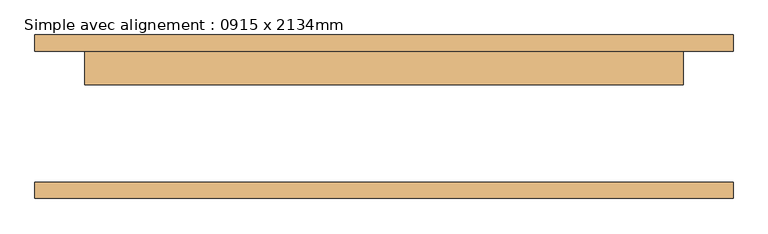
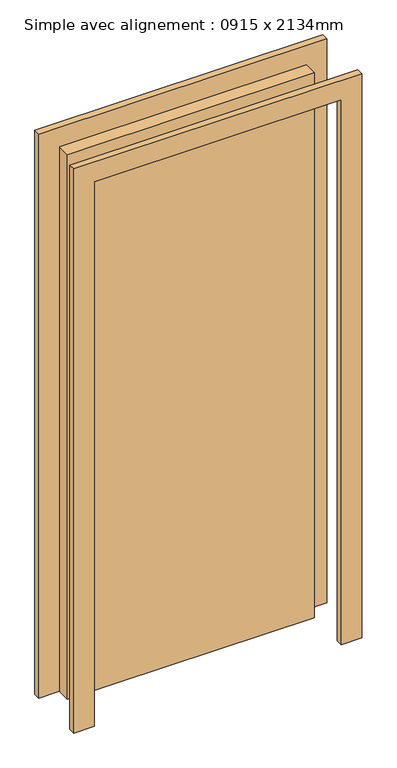
"""IFC4 building model written with IfcOpenShell, lengths in millimetres: door geometry, Simple avec alignement : 0915 x 2134mm."""

from ifc_helpers import new_model, si_unit, frame, origin, origin_with_axes, place, context, project, spatial, polyline, outline, extrude, source, transform, mapped, element, save


def simple_avec_alignement_0915_x_2134mm_6a9e8738(model_context):
    return source(origin(), model_context, "Body", "SweptSolid", [
        extrude(outline(polyline([(2210.0, -533.5), (0.0, -533.5), (0.0, -457.5), (2134.0, -457.5), (2134.0, 457.5), (0.0, 457.5), (0.0, 533.5), (2210.0, 533.5), (2210.0, -533.5)])), frame((0.0, 100.0, 0.0), z_axis=(0.0, 1.0, 0.0), x_axis=(0.0, 0.0, 1.0)), (0.0, 0.0, 1.0), 25.0),
        extrude(outline(polyline([(2210.0, 533.5), (2210.0, -533.5), (0.0, -533.5), (0.0, -457.5), (2134.0, -457.5), (2134.0, 457.5), (0.0, 457.5), (0.0, 533.5), (2210.0, 533.5)])), frame((0.0, -125.0, 0.0), z_axis=(0.0, 1.0, 0.0), x_axis=(0.0, 0.0, 1.0)), (0.0, 0.0, 1.0), 25.0),
        extrude(outline(polyline([(457.5, 49.0), (-457.5, 49.0), (-457.5, 100.0), (457.5, 100.0), (457.5, 49.0)])), origin_with_axes(), (0.0, 0.0, 1.0), 2134.0),
    ])


if __name__ == "__main__":
    model = new_model("IFC4")
    model_context = context("Model", 3, world=origin())
    ifc_project = project(units=[si_unit("LENGTHUNIT", "METRE", prefix="MILLI")], contexts=[model_context])
    site = spatial("IfcSite", under=ifc_project)
    building = spatial("IfcBuilding", under=site)
    placement = place(None, origin())
    simple_avec_alignement_0915_x_2134mm_shape = simple_avec_alignement_0915_x_2134mm_6a9e8738(model_context)
    element("IfcDoor", 1, ObjectType="Simple avec alignement : 0915 x 2134mm", at=placement, inside=building, context=model_context, shape_type="MappedRepresentation", body=[
        mapped(simple_avec_alignement_0915_x_2134mm_shape, transform((0.0, 0.0, 0.0), x_axis=(1.0, 0.0, 0.0), y_axis=(0.0, 1.0, 0.0), z_axis=(0.0, 0.0, 1.0))),
    ])
    save(model, "model.ifc")

# Revit data of these elements
# Type "Simple avec alignement : 0915 x 2134mm"
#   Type Mark = "10"
#   Construction Type Id = "MDOOR"
#   Analytic Construction = "Métal"
#   Thickness = 0.051 m
#   Heat Transfer Coefficient (U) = 3.7021 W/(m²·K)
#   Height = 2.134 m
#   Ajuster la projection Ext = 0.025 m
#   Ajuster la projection Int = 0.025 m
#   Ajuster la largeur = 0.076 m
#   Width = 0.915 m
#   Function = 0
#   Define Thermal Properties by = 1
#   Matériau de porte = Porte - Panneau
#   Matériau des huisseries = Porte - Cadre
#   Visual Light Transmittance = 0
#   Solar Heat Gain Coefficient = 0
#   Function = (empty or 0)
#   Wall Closure = (empty or 0)
# Element 1 (IfcDoor, "Simple avec alignement : 0915 x 2134mm")
#   Materials on its faces: "Porte - Cadre", "Porte - Panneau"
# Materials
#   "Porte - Panneau": class "Bois", colour RGB 210 159 95, transparency 0, Cost = 0
#   "Porte - Cadre": class "Peinture", colour RGB 118 70 51, transparency 0, Cost = 0
